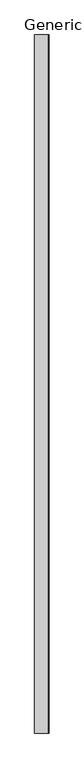
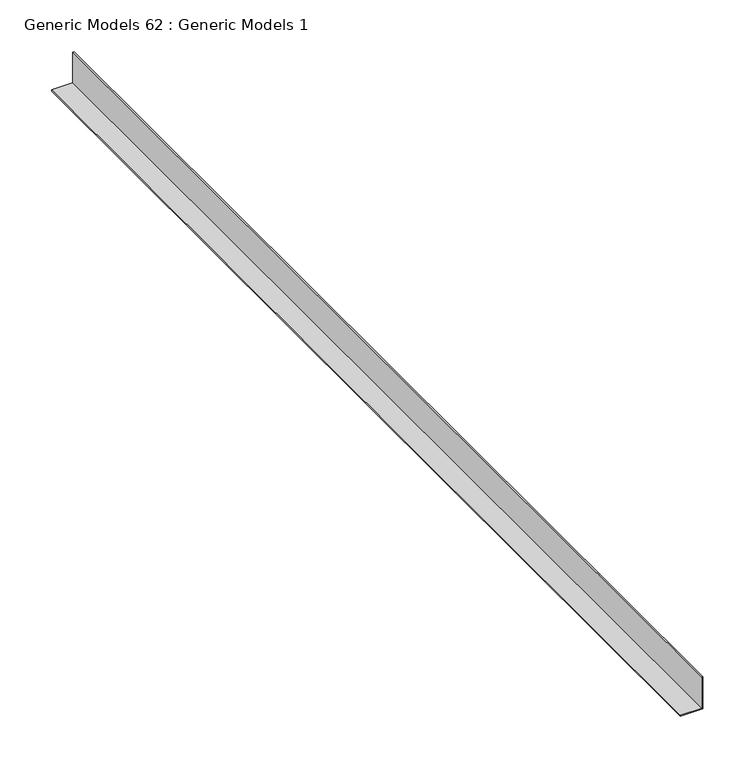
"""IFC4 building model written with IfcOpenShell, lengths in millimetres: proxy geometry, Generic Models 62 : Generic Models 1."""

import ifcopenshell
import ifcopenshell.guid

model = None  # the IFC model being written
_history = None  # IfcOwnerHistory: only IFC2X3 demands one
_inside = {}  # id of a spatial element -> (the spatial element, [elements in it])
_under = {}  # id of a project, library or spatial element -> (it, [spatial elements below it])
_declared = {}  # id of a project -> (the project, [libraries it declares])
_typed = {}  # id of a type object -> (the type object, [elements of that type])
_made_of = {}  # id of a material, layer set ... -> (it, [elements and type objects made of it])


def new_model(schema):
    """Start an empty IFC model of exactly this schema.

    Asked for "IFC4X3", IfcOpenShell would pick the latest addendum, in which some entities
    have other attributes; the version numbers below select the first issue.
    IFC2X3 requires an IfcOwnerHistory on every rooted entity: one is made here for all.
    """
    global model, _history
    if schema == "IFC4X3":
        model = ifcopenshell.file(schema_version=(4, 3, 0, 0))
    else:
        model = ifcopenshell.file(schema=schema)
    _inside.clear()
    _under.clear()
    _declared.clear()
    _typed.clear()
    _made_of.clear()
    _history = None
    if model.schema == "IFC2X3":
        org = make("IfcOrganization", Name="unknown")
        user = make(
            "IfcPersonAndOrganization",
            ThePerson=make("IfcPerson", FamilyName="unknown"),
            TheOrganization=org,
        )
        app = make(
            "IfcApplication",
            ApplicationDeveloper=org,
            Version="unknown",
            ApplicationFullName="unknown",
            ApplicationIdentifier="unknown",
        )
        _history = make(
            "IfcOwnerHistory",
            OwningUser=user,
            OwningApplication=app,
            ChangeAction="ADDED",
            CreationDate=0,
        )
    return model


def make(cls, **values):
    """One entity of the class cls with the attributes given. An attribute that is None is left unset."""
    return model.create_entity(
        cls, **{name: value for name, value in values.items() if value is not None}
    )


def rooted(cls, **values):
    """An entity with a GlobalId (a new one), such as an element, a storey or a relation."""
    return make(cls, GlobalId=ifcopenshell.guid.new(), OwnerHistory=_history, **values)


def si_unit(unit_type, name, prefix=None):
    """IfcSIUnit, for example si_unit("LENGTHUNIT", "METRE", prefix="MILLI")."""
    return make("IfcSIUnit", UnitType=unit_type, Prefix=prefix, Name=name)


def assignment(units):
    """IfcUnitAssignment: the units of a project."""
    return None if units is None else make("IfcUnitAssignment", Units=units)


def point(xyz):
    """IfcCartesianPoint."""
    return None if xyz is None else make("IfcCartesianPoint", Coordinates=xyz)


def direction(xyz):
    """IfcDirection."""
    return None if xyz is None else make("IfcDirection", DirectionRatios=xyz)


def frame(location, z_axis=None, x_axis=None):
    """IfcAxis2Placement3D, a coordinate frame: its origin and axes. An axis left out is left unset."""
    return make(
        "IfcAxis2Placement3D",
        Location=point(location),
        Axis=direction(z_axis),
        RefDirection=direction(x_axis),
    )


def origin():
    """The frame at (0, 0, 0) with its axes left unset."""
    return frame((0.0, 0.0, 0.0))


def place(relative_to, where):
    """IfcLocalPlacement: puts the frame where relative to a parent placement (None: the world)."""
    return make(
        "IfcLocalPlacement", PlacementRelTo=relative_to, RelativePlacement=where
    )


def context(
    kind, dimensions, precision=None, world=None, true_north=None, identifier=None
):
    """IfcGeometricRepresentationContext, for example the 3D "Model" context."""
    return make(
        "IfcGeometricRepresentationContext",
        ContextIdentifier=identifier,
        ContextType=kind,
        CoordinateSpaceDimension=dimensions,
        Precision=precision,
        WorldCoordinateSystem=world,
        TrueNorth=true_north,
    )


def project(units=None, contexts=None):
    """IfcProject with its units and contexts."""
    return rooted(
        "IfcProject",
        Name="project",
        RepresentationContexts=contexts,
        UnitsInContext=assignment(units),
    )


def spatial(cls, under=None, at=None, **own):
    """A site, building, storey or space (cls), placed at a placement, below another one or the project."""
    s = rooted(cls, ObjectPlacement=at, **own)
    if under is not None:
        _under.setdefault(under.id(), (under, []))[1].append(s)
    return s


def polyline(points):
    """IfcPolyline through the points."""
    return make("IfcPolyline", Points=[point(p) for p in points])


def outline(outer, holes=None, kind="AREA"):
    """IfcArbitraryClosedProfileDef: a profile drawn as a closed curve; with holes, ...WithVoids."""
    if holes is None:
        return make("IfcArbitraryClosedProfileDef", ProfileType=kind, OuterCurve=outer)
    return make(
        "IfcArbitraryProfileDefWithVoids",
        ProfileType=kind,
        OuterCurve=outer,
        InnerCurves=holes,
    )


def extrude(swept, where, along, depth):
    """IfcExtrudedAreaSolid: the profile swept, set in the frame where, extruded along a direction by depth."""
    return make(
        "IfcExtrudedAreaSolid",
        SweptArea=swept,
        Position=where,
        ExtrudedDirection=direction(along),
        Depth=depth,
    )


def shape(context_of_items, identifier, shape_type, items):
    """IfcShapeRepresentation: the items that make up one representation, for example the "Body"."""
    return make(
        "IfcShapeRepresentation",
        ContextOfItems=context_of_items,
        RepresentationIdentifier=identifier,
        RepresentationType=shape_type,
        Items=items,
    )


def source(mapping_origin, context_of_items, identifier, shape_type, items):
    """IfcRepresentationMap: a shape defined once, which mapped items show again and again."""
    return make(
        "IfcRepresentationMap",
        MappingOrigin=mapping_origin,
        MappedRepresentation=shape(context_of_items, identifier, shape_type, items),
    )


def transform(
    local_origin,
    x_axis=None,
    y_axis=None,
    z_axis=None,
    scale=None,
    scale2=None,
    scale3=None,
    uniform=True,
):
    """IfcCartesianTransformationOperator3D, or its non-uniform kind. x_axis, y_axis, z_axis: its Axis1, 2, 3."""
    if uniform:
        return make(
            "IfcCartesianTransformationOperator3D",
            Axis1=direction(x_axis),
            Axis2=direction(y_axis),
            LocalOrigin=point(local_origin),
            Scale=scale,
            Axis3=direction(z_axis),
        )
    return make(
        "IfcCartesianTransformationOperator3DnonUniform",
        Axis1=direction(x_axis),
        Axis2=direction(y_axis),
        LocalOrigin=point(local_origin),
        Scale=scale,
        Axis3=direction(z_axis),
        Scale2=scale2,
        Scale3=scale3,
    )


def mapped(mapping_source, mapping_target):
    """IfcMappedItem: shows the shape of a source again, moved by a transform."""
    return make(
        "IfcMappedItem", MappingSource=mapping_source, MappingTarget=mapping_target
    )


def made_of(thing, what):
    """Note that an element or type object is made of a material, layer set ...; save() writes the relation."""
    if what is not None:
        _made_of.setdefault(what.id(), (what, []))[1].append(thing)
    return thing


def element(
    cls,
    number,
    at=None,
    inside=None,
    cuts=None,
    type_object=None,
    material=None,
    context=None,
    identifier="Body",
    shape_type=None,
    held_by="IfcProductDefinitionShape",
    body=None,
    shapes=None,
    **own,
):
    """One element of the class cls, such as IfcWall. Its Tag is "e" and its number.

    at: its placement. inside: the storey or other place that contains it. cuts: it is an
    opening in that element (IfcRelVoidsElement). A single representation is given by context,
    identifier, shape_type and body (its items); several are given by shapes. held_by: the class
    of the entity that holds the representations. save() writes the other relations.
    """
    e = rooted(cls, Tag="e%d" % number, ObjectPlacement=at, **own)
    if body is not None:
        shapes = [shape(context, identifier, shape_type, body)]
    if shapes is not None:
        e.Representation = make(held_by, Representations=shapes)
    if inside is not None:
        _inside.setdefault(inside.id(), (inside, []))[1].append(e)
    if cuts is not None:
        rooted(
            "IfcRelVoidsElement", RelatingBuildingElement=cuts, RelatedOpeningElement=e
        )
    if type_object is not None:
        _typed.setdefault(type_object.id(), (type_object, []))[1].append(e)
    return made_of(e, material)


def aggregate(whole, parts):
    """IfcRelAggregates: a whole, such as a stair, and the parts it consists of."""
    return rooted("IfcRelAggregates", RelatingObject=whole, RelatedObjects=parts)


def save(model, path):
    """Write the relations noted so far, then the file.

    IfcRelAggregates (storeys below a building ...), IfcRelContainedInSpatialStructure (elements
    in a storey), IfcRelDefinesByType, IfcRelAssociatesMaterial and IfcRelDeclares: one each for
    every whole, place, type object, material and project.
    """
    for whole, parts in _under.values():
        aggregate(whole, parts)
    for where, things in _inside.values():
        rooted(
            "IfcRelContainedInSpatialStructure",
            RelatedElements=things,
            RelatingStructure=where,
        )
    for kind, things in _typed.values():
        rooted("IfcRelDefinesByType", RelatedObjects=things, RelatingType=kind)
    for what, things in _made_of.values():
        rooted("IfcRelAssociatesMaterial", RelatedObjects=things, RelatingMaterial=what)
    for by, libraries in _declared.values():
        rooted("IfcRelDeclares", RelatingContext=by, RelatedDefinitions=libraries)
    model.write(path)


def generic_models_62_generic_models_1_528f8659(model_context):
    return source(origin(), model_context, "Body", "SweptSolid", [
        extrude(outline(polyline([(2277.1204978, 51991.1377541), (2277.1204978, 51989.5502541), (2240.6079978, 51989.5502541), (2240.6079978, 51965.7377541), (2239.0204978, 51965.7377541), (2239.0204978, 51991.1377541), (2277.1204978, 51991.1377541)])), frame((0.0, 0.0, 0.0), z_axis=(0.0, 1.0, 0.0), x_axis=(0.0, 0.0, 1.0)), (0.0, 0.0, 1.0), 1219.2),
    ])


if __name__ == "__main__":
    model = new_model("IFC4")
    model_context = context("Model", 3, world=origin())
    ifc_project = project(units=[si_unit("LENGTHUNIT", "METRE", prefix="MILLI")], contexts=[model_context])
    site = spatial("IfcSite", under=ifc_project)
    building = spatial("IfcBuilding", under=site)
    placement = place(None, origin())
    generic_models_62_generic_models_1_shape = generic_models_62_generic_models_1_528f8659(model_context)
    element("IfcBuildingElementProxy", 1, Name="Generic Models 62 : Generic Models 1", ObjectType="Generic Models 62 : Generic Models 1", at=placement, inside=building, context=model_context, shape_type="MappedRepresentation", body=[
        mapped(generic_models_62_generic_models_1_shape, transform((0.0, 0.0, 0.0), x_axis=(1.0, 0.0, 0.0), y_axis=(0.0, 1.0, 0.0), z_axis=(0.0, 0.0, 1.0))),
    ])
    save(model, "model.ifc")

# Revit data of these elements
# Element 1 (IfcBuildingElementProxy, "Generic Models 62 : Generic Models 1")
#   Materials on its faces: "CEILING TRACK AS SCHEDULED"
# Materials
#   "CEILING TRACK AS SCHEDULED": class "Unassigned", colour RGB 210 209 208, transparency 0, Keynote = "M05121300.02", Cost = 0
